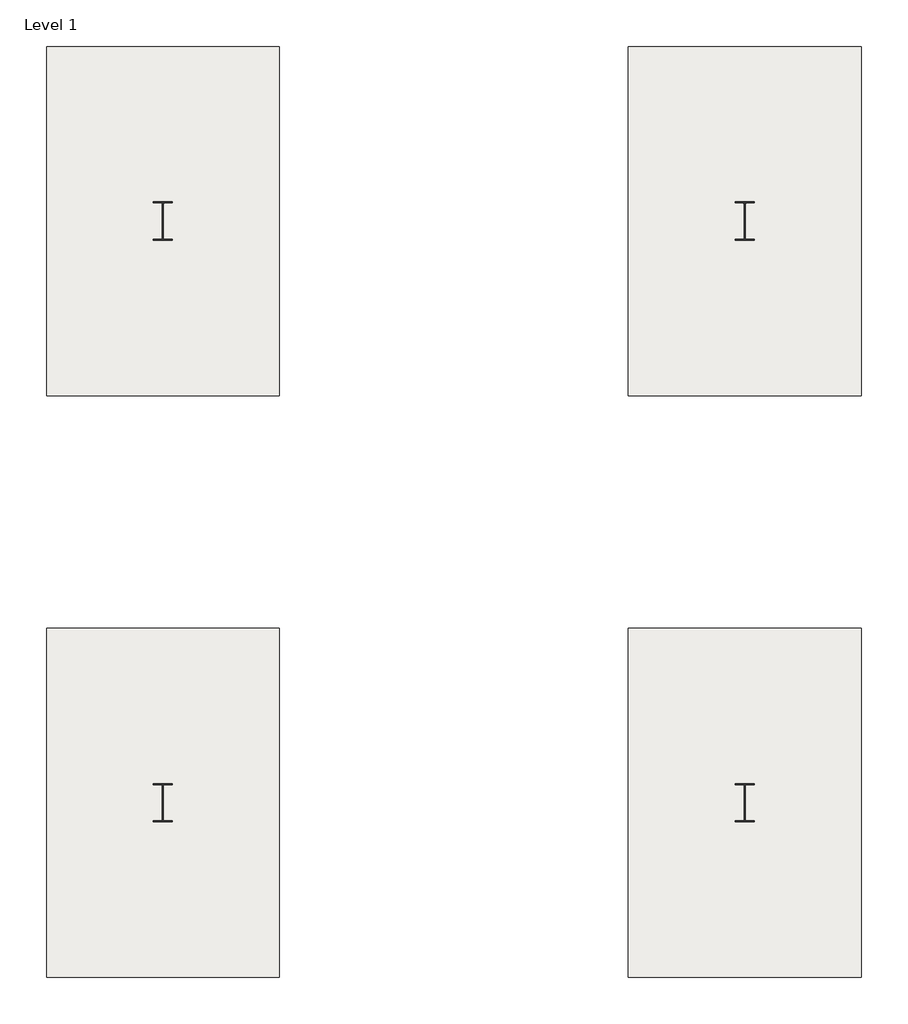
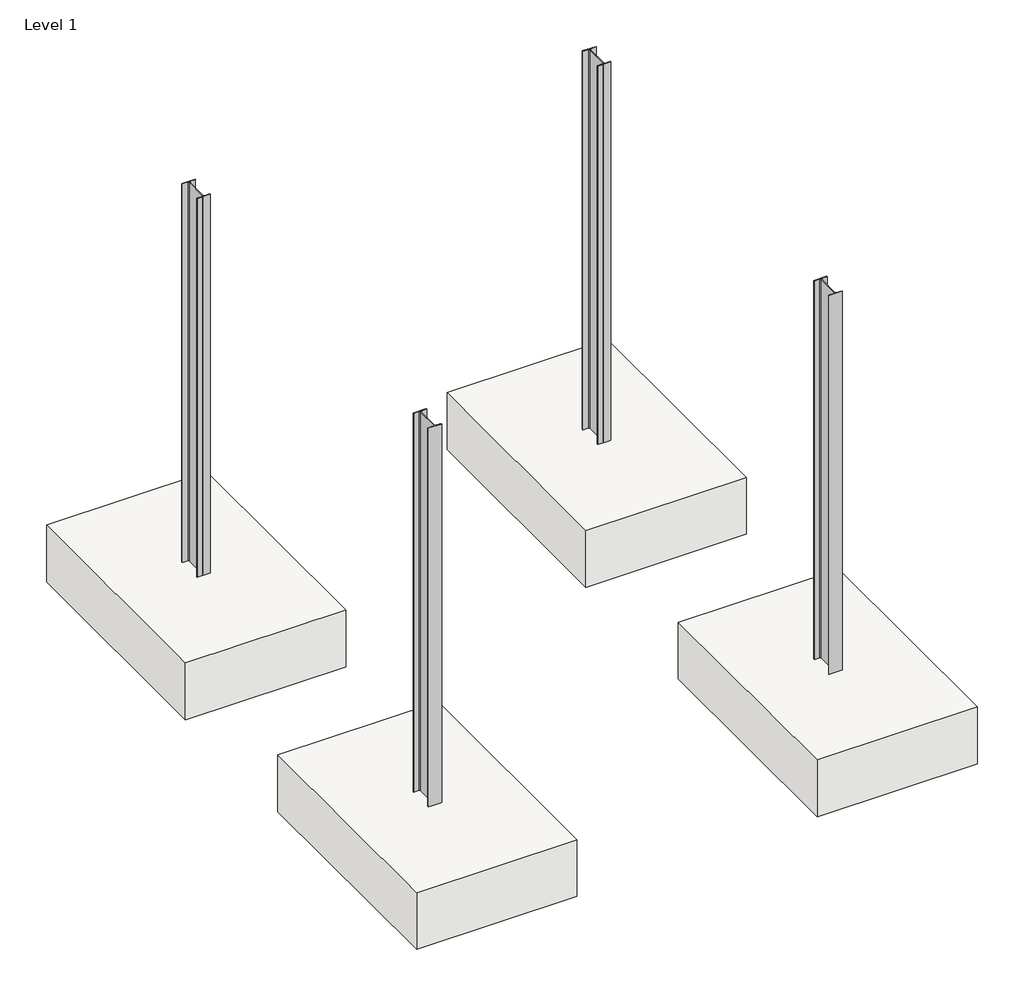
# One storey: 4 columns, 4 slabs.
"""IFC4 building model written with IfcOpenShell, lengths in millimetres."""

import ifcopenshell
import ifcopenshell.guid

model = None  # the IFC model being written
_history = None  # IfcOwnerHistory: only IFC2X3 demands one
_inside = {}  # id of a spatial element -> (the spatial element, [elements in it])
_under = {}  # id of a project, library or spatial element -> (it, [spatial elements below it])
_declared = {}  # id of a project -> (the project, [libraries it declares])
_typed = {}  # id of a type object -> (the type object, [elements of that type])
_made_of = {}  # id of a material, layer set ... -> (it, [elements and type objects made of it])


def new_model(schema):
    """Start an empty IFC model of exactly this schema.

    Asked for "IFC4X3", IfcOpenShell would pick the latest addendum, in which some entities
    have other attributes; the version numbers below select the first issue.
    IFC2X3 requires an IfcOwnerHistory on every rooted entity: one is made here for all.
    """
    global model, _history
    if schema == "IFC4X3":
        model = ifcopenshell.file(schema_version=(4, 3, 0, 0))
    else:
        model = ifcopenshell.file(schema=schema)
    _inside.clear()
    _under.clear()
    _declared.clear()
    _typed.clear()
    _made_of.clear()
    _history = None
    if model.schema == "IFC2X3":
        org = make("IfcOrganization", Name="unknown")
        user = make(
            "IfcPersonAndOrganization",
            ThePerson=make("IfcPerson", FamilyName="unknown"),
            TheOrganization=org,
        )
        app = make(
            "IfcApplication",
            ApplicationDeveloper=org,
            Version="unknown",
            ApplicationFullName="unknown",
            ApplicationIdentifier="unknown",
        )
        _history = make(
            "IfcOwnerHistory",
            OwningUser=user,
            OwningApplication=app,
            ChangeAction="ADDED",
            CreationDate=0,
        )
    return model


def make(cls, **values):
    """One entity of the class cls with the attributes given. An attribute that is None is left unset."""
    return model.create_entity(
        cls, **{name: value for name, value in values.items() if value is not None}
    )


def rooted(cls, **values):
    """An entity with a GlobalId (a new one), such as an element, a storey or a relation."""
    return make(cls, GlobalId=ifcopenshell.guid.new(), OwnerHistory=_history, **values)


def si_unit(unit_type, name, prefix=None):
    """IfcSIUnit, for example si_unit("LENGTHUNIT", "METRE", prefix="MILLI")."""
    return make("IfcSIUnit", UnitType=unit_type, Prefix=prefix, Name=name)


def assignment(units):
    """IfcUnitAssignment: the units of a project."""
    return None if units is None else make("IfcUnitAssignment", Units=units)


def point(xyz):
    """IfcCartesianPoint."""
    return None if xyz is None else make("IfcCartesianPoint", Coordinates=xyz)


def direction(xyz):
    """IfcDirection."""
    return None if xyz is None else make("IfcDirection", DirectionRatios=xyz)


def frame(location, z_axis=None, x_axis=None):
    """IfcAxis2Placement3D, a coordinate frame: its origin and axes. An axis left out is left unset."""
    return make(
        "IfcAxis2Placement3D",
        Location=point(location),
        Axis=direction(z_axis),
        RefDirection=direction(x_axis),
    )


def frame_2d(location, x_axis=None):
    """IfcAxis2Placement2D, a coordinate frame in the plane: its origin and x axis."""
    return make(
        "IfcAxis2Placement2D", Location=point(location), RefDirection=direction(x_axis)
    )


def origin():
    """The frame at (0, 0, 0) with its axes left unset."""
    return frame((0.0, 0.0, 0.0))


def origin_with_axes():
    """The frame at (0, 0, 0) with the z axis (0, 0, 1) and the x axis (1, 0, 0) written out."""
    return frame((0.0, 0.0, 0.0), z_axis=(0.0, 0.0, 1.0), x_axis=(1.0, 0.0, 0.0))


def place(relative_to, where):
    """IfcLocalPlacement: puts the frame where relative to a parent placement (None: the world)."""
    return make(
        "IfcLocalPlacement", PlacementRelTo=relative_to, RelativePlacement=where
    )


def context(
    kind, dimensions, precision=None, world=None, true_north=None, identifier=None
):
    """IfcGeometricRepresentationContext, for example the 3D "Model" context."""
    return make(
        "IfcGeometricRepresentationContext",
        ContextIdentifier=identifier,
        ContextType=kind,
        CoordinateSpaceDimension=dimensions,
        Precision=precision,
        WorldCoordinateSystem=world,
        TrueNorth=true_north,
    )


def project(units=None, contexts=None):
    """IfcProject with its units and contexts."""
    return rooted(
        "IfcProject",
        Name="project",
        RepresentationContexts=contexts,
        UnitsInContext=assignment(units),
    )


def spatial(cls, under=None, at=None, **own):
    """A site, building, storey or space (cls), placed at a placement, below another one or the project."""
    s = rooted(cls, ObjectPlacement=at, **own)
    if under is not None:
        _under.setdefault(under.id(), (under, []))[1].append(s)
    return s


def polyline(points):
    """IfcPolyline through the points."""
    return make("IfcPolyline", Points=[point(p) for p in points])


def circle_curve(where, radius):
    """IfcCircle in the frame where."""
    return make("IfcCircle", Position=where, Radius=radius)


def trimmed(basis, trim1, trim2, sense, master):
    """IfcTrimmedCurve: the piece of a basis curve between two trims."""
    return make(
        "IfcTrimmedCurve",
        BasisCurve=basis,
        Trim1=trim1,
        Trim2=trim2,
        SenseAgreement=sense,
        MasterRepresentation=master,
    )


def segment(curve, same_sense, transition):
    """IfcCompositeCurveSegment."""
    return make(
        "IfcCompositeCurveSegment",
        Transition=transition,
        SameSense=same_sense,
        ParentCurve=curve,
    )


def composite_curve(segments, self_intersect=None):
    """IfcCompositeCurve: segments joined end to end."""
    return make("IfcCompositeCurve", Segments=segments, SelfIntersect=self_intersect)


def outline(outer, holes=None, kind="AREA"):
    """IfcArbitraryClosedProfileDef: a profile drawn as a closed curve; with holes, ...WithVoids."""
    if holes is None:
        return make("IfcArbitraryClosedProfileDef", ProfileType=kind, OuterCurve=outer)
    return make(
        "IfcArbitraryProfileDefWithVoids",
        ProfileType=kind,
        OuterCurve=outer,
        InnerCurves=holes,
    )


def extrude(swept, where, along, depth):
    """IfcExtrudedAreaSolid: the profile swept, set in the frame where, extruded along a direction by depth."""
    return make(
        "IfcExtrudedAreaSolid",
        SweptArea=swept,
        Position=where,
        ExtrudedDirection=direction(along),
        Depth=depth,
    )


def shape(context_of_items, identifier, shape_type, items):
    """IfcShapeRepresentation: the items that make up one representation, for example the "Body"."""
    return make(
        "IfcShapeRepresentation",
        ContextOfItems=context_of_items,
        RepresentationIdentifier=identifier,
        RepresentationType=shape_type,
        Items=items,
    )


def source(mapping_origin, context_of_items, identifier, shape_type, items):
    """IfcRepresentationMap: a shape defined once, which mapped items show again and again."""
    return make(
        "IfcRepresentationMap",
        MappingOrigin=mapping_origin,
        MappedRepresentation=shape(context_of_items, identifier, shape_type, items),
    )


def transform(
    local_origin,
    x_axis=None,
    y_axis=None,
    z_axis=None,
    scale=None,
    scale2=None,
    scale3=None,
    uniform=True,
):
    """IfcCartesianTransformationOperator3D, or its non-uniform kind. x_axis, y_axis, z_axis: its Axis1, 2, 3."""
    if uniform:
        return make(
            "IfcCartesianTransformationOperator3D",
            Axis1=direction(x_axis),
            Axis2=direction(y_axis),
            LocalOrigin=point(local_origin),
            Scale=scale,
            Axis3=direction(z_axis),
        )
    return make(
        "IfcCartesianTransformationOperator3DnonUniform",
        Axis1=direction(x_axis),
        Axis2=direction(y_axis),
        LocalOrigin=point(local_origin),
        Scale=scale,
        Axis3=direction(z_axis),
        Scale2=scale2,
        Scale3=scale3,
    )


def mapped(mapping_source, mapping_target):
    """IfcMappedItem: shows the shape of a source again, moved by a transform."""
    return make(
        "IfcMappedItem", MappingSource=mapping_source, MappingTarget=mapping_target
    )


def made_of(thing, what):
    """Note that an element or type object is made of a material, layer set ...; save() writes the relation."""
    if what is not None:
        _made_of.setdefault(what.id(), (what, []))[1].append(thing)
    return thing


def element(
    cls,
    number,
    at=None,
    inside=None,
    cuts=None,
    type_object=None,
    material=None,
    context=None,
    identifier="Body",
    shape_type=None,
    held_by="IfcProductDefinitionShape",
    body=None,
    shapes=None,
    **own,
):
    """One element of the class cls, such as IfcWall. Its Tag is "e" and its number.

    at: its placement. inside: the storey or other place that contains it. cuts: it is an
    opening in that element (IfcRelVoidsElement). A single representation is given by context,
    identifier, shape_type and body (its items); several are given by shapes. held_by: the class
    of the entity that holds the representations. save() writes the other relations.
    """
    e = rooted(cls, Tag="e%d" % number, ObjectPlacement=at, **own)
    if body is not None:
        shapes = [shape(context, identifier, shape_type, body)]
    if shapes is not None:
        e.Representation = make(held_by, Representations=shapes)
    if inside is not None:
        _inside.setdefault(inside.id(), (inside, []))[1].append(e)
    if cuts is not None:
        rooted(
            "IfcRelVoidsElement", RelatingBuildingElement=cuts, RelatedOpeningElement=e
        )
    if type_object is not None:
        _typed.setdefault(type_object.id(), (type_object, []))[1].append(e)
    return made_of(e, material)


def aggregate(whole, parts):
    """IfcRelAggregates: a whole, such as a stair, and the parts it consists of."""
    return rooted("IfcRelAggregates", RelatingObject=whole, RelatedObjects=parts)


def save(model, path):
    """Write the relations noted so far, then the file.

    IfcRelAggregates (storeys below a building ...), IfcRelContainedInSpatialStructure (elements
    in a storey), IfcRelDefinesByType, IfcRelAssociatesMaterial and IfcRelDeclares: one each for
    every whole, place, type object, material and project.
    """
    for whole, parts in _under.values():
        aggregate(whole, parts)
    for where, things in _inside.values():
        rooted(
            "IfcRelContainedInSpatialStructure",
            RelatedElements=things,
            RelatingStructure=where,
        )
    for kind, things in _typed.values():
        rooted("IfcRelDefinesByType", RelatedObjects=things, RelatingType=kind)
    for what, things in _made_of.values():
        rooted("IfcRelAssociatesMaterial", RelatedObjects=things, RelatingMaterial=what)
    for by, libraries in _declared.values():
        rooted("IfcRelDeclares", RelatingContext=by, RelatedDefinitions=libraries)
    model.write(path)


def w_shapes_column_w8x10_fd6cb265(model_context):
    return source(origin(), model_context, "Body", "SweptSolid", [
        extrude(outline(composite_curve([segment(polyline([(50.038, 100.203), (50.038, 94.869), (9.779, 94.869)]), True, "CONTINUOUS"), segment(trimmed(circle_curve(frame_2d((9.779, 87.249)), 7.62), [point((9.779, 94.869))], [point((2.159, 87.249))], True, "CARTESIAN"), True, "CONTINUOUS"), segment(polyline([(2.159, 87.249), (2.159, -87.249)]), True, "CONTINUOUS"), segment(trimmed(circle_curve(frame_2d((9.779, -87.249)), 7.62), [point((2.159, -87.249))], [point((9.779, -94.869))], True, "CARTESIAN"), True, "CONTINUOUS"), segment(polyline([(9.779, -94.869), (50.038, -94.869), (50.038, -100.203), (-50.038, -100.203), (-50.038, -94.869), (-9.779, -94.869)]), True, "CONTINUOUS"), segment(trimmed(circle_curve(frame_2d((-9.779, -87.249)), 7.62), [point((-9.779, -94.869))], [point((-2.159, -87.249))], True, "CARTESIAN"), True, "CONTINUOUS"), segment(polyline([(-2.159, -87.249), (-2.159, 87.249)]), True, "CONTINUOUS"), segment(trimmed(circle_curve(frame_2d((-9.779, 87.249)), 7.62), [point((-2.159, 87.249))], [point((-9.779, 94.869))], True, "CARTESIAN"), True, "CONTINUOUS"), segment(polyline([(-9.779, 94.869), (-50.038, 94.869), (-50.038, 100.203), (50.038, 100.203)]), True, "CONTINUOUS")], self_intersect=False)), origin_with_axes(), (0.0, 0.0, 1.0), 3048.0),
    ])


def slab_5ba74754(model_context):
    return source(origin(), model_context, "Body", "SweptSolid", [
        extrude(outline(polyline([(609.6, 914.4), (609.6, -914.4), (-609.6, -914.4), (-609.6, 914.4), (609.6, 914.4)])), frame((0.0, 0.0, -457.2), z_axis=(0.0, 0.0, 1.0), x_axis=(1.0, 0.0, 0.0)), (0.0, 0.0, 1.0), 457.2),
    ])


model = new_model("IFC4")

# Units and contexts
model_context = context("Model", 3, world=origin())
ifc_project = project(units=[si_unit("LENGTHUNIT", "METRE", prefix="MILLI")], contexts=[model_context])

# Site, building, storey
site = spatial("IfcSite", under=ifc_project)
building = spatial("IfcBuilding", under=site)
storey = spatial("IfcBuildingStorey", under=building, Name="Level 1", Elevation=0.0)

# Columns
placement = place(None, origin())
w_shapes_column_w8x10_shape = w_shapes_column_w8x10_fd6cb265(model_context)
element("IfcColumn", 1, ObjectType="W Shapes-Column : W8X10", at=placement, inside=storey, context=model_context, shape_type="MappedRepresentation", body=[
    mapped(w_shapes_column_w8x10_shape, transform((3048.0, 0.0, 0.0), x_axis=(1.0, 0.0, 0.0), y_axis=(0.0, 1.0, 0.0), z_axis=(0.0, 0.0, 1.0))),
])
element("IfcColumn", 2, ObjectType="W Shapes-Column : W8X10", at=placement, inside=storey, context=model_context, shape_type="MappedRepresentation", body=[
    mapped(w_shapes_column_w8x10_shape, transform((3048.0, 3048.0, 0.0), x_axis=(1.0, 0.0, 0.0), y_axis=(0.0, 1.0, 0.0), z_axis=(0.0, 0.0, 1.0))),
])
element("IfcColumn", 3, ObjectType="W Shapes-Column : W8X10", at=placement, inside=storey, context=model_context, shape_type="MappedRepresentation", body=[
    mapped(w_shapes_column_w8x10_shape, transform((0.0, 3048.0, 0.0), x_axis=(1.0, 0.0, 0.0), y_axis=(0.0, 1.0, 0.0), z_axis=(0.0, 0.0, 1.0))),
])
element("IfcColumn", 4, ObjectType="W Shapes-Column : W8X10", at=placement, inside=storey, context=model_context, shape_type="MappedRepresentation", body=[
    mapped(w_shapes_column_w8x10_shape, transform((0.0, 0.0, 0.0), x_axis=(1.0, 0.0, 0.0), y_axis=(0.0, 1.0, 0.0), z_axis=(0.0, 0.0, 1.0))),
])

# Slabs
slab_shape = slab_5ba74754(model_context)
element("IfcSlab", 5, ObjectType="Footing-Rectangular : 72\" x 48\" x 18\"", at=placement, inside=storey, context=model_context, shape_type="MappedRepresentation", body=[
    mapped(slab_shape, transform((0.0, 3048.0, 0.0), x_axis=(1.0, 0.0, 0.0), y_axis=(0.0, 1.0, 0.0), z_axis=(0.0, 0.0, 1.0))),
])
element("IfcSlab", 6, ObjectType="Footing-Rectangular : 72\" x 48\" x 18\"", at=placement, inside=storey, context=model_context, shape_type="MappedRepresentation", body=[
    mapped(slab_shape, transform((3048.0, 3048.0, 0.0), x_axis=(1.0, 0.0, 0.0), y_axis=(0.0, 1.0, 0.0), z_axis=(0.0, 0.0, 1.0))),
])
element("IfcSlab", 7, ObjectType="Footing-Rectangular : 72\" x 48\" x 18\"", at=placement, inside=storey, context=model_context, shape_type="MappedRepresentation", body=[
    mapped(slab_shape, transform((3048.0, 0.0, 0.0), x_axis=(1.0, 0.0, 0.0), y_axis=(0.0, 1.0, 0.0), z_axis=(0.0, 0.0, 1.0))),
])
element("IfcSlab", 8, ObjectType="Footing-Rectangular : 72\" x 48\" x 18\"", at=placement, inside=storey, context=model_context, shape_type="MappedRepresentation", body=[
    mapped(slab_shape, transform((0.0, 0.0, 0.0), x_axis=(1.0, 0.0, 0.0), y_axis=(0.0, 1.0, 0.0), z_axis=(0.0, 0.0, 1.0))),
])

save(model, "model.ifc")

# Revit data of these elements
# Project information
#   Project Issue Date = "Issue Date"
#   Project Status = "Project Status"
#   Client Name = "Owner"
#   Project Address = "Enter address here"
#   Project Name = "Project Name"
#   Project Number = "Project Number"
# Grids (mm)
#   "1": line (0, 3382.905) -> (0, -500.676)
#   "2": line (3048, 3382.905) -> (3048, -500.676)
#   "B": line (3628.947, 0) -> (-577.435, 0)
#   "A": line (3628.947, 3048) -> (-577.435, 3048)
# Type "W Shapes-Column : W8X10"
#   Section Name Key = "W8x10"
#   Assembly Code = "B10"
#   Width = 100.076 mm
#   Web Thickness = 4.318 mm
#   Web Fillet = 7.62 mm
#   Warping Constant = 8297.76 cm⁶
#   Torsional Moment of Inertia = 1.77315 cm⁴
#   Section Area = 2.96 in²
#   Plastic Modulus weak axis = 0.000960648 (stored number, unit not read)
#   Plastic Modulus strong axis = 0.0051331 (stored number, unit not read)
#   Perimeter = 9.35736 m²/m
#   Nominal Weight = 145.939 N/m
#   Moment of Inertia weak axis = 86.9924 cm⁴
#   Moment of Inertia strong axis = 1281.99 cm⁴
#   Height = 200.406 mm
#   Flange Thickness = 5.334 mm
#   Elastic Modulus weak axis = 0.000613426 (stored number, unit not read)
#   Elastic Modulus strong axis = 0.00451968 (stored number, unit not read)
#   Centroid Vertical = 100.203 mm
#   Centroid Horizontal = 50.038 mm
#   Structural Material [instance default] = Steel ASTM A992
#   Principal Axes Angle = 0
# Type "Footing-Rectangular : 72\" x 48\" x 18\""
#   Assembly Code = "A1010100"
#   Width = 4' - 0"
#   Length = 6' - 0"
#   Thickness = 1' - 6"
#   Structural Material [instance default] = Concrete, Cast-in-Place gray
# Elements 1, 2, 3, 4 (IfcColumn, "W Shapes-Column : W8X10")
#   Comments = ""
#   Structural Material = Steel ASTM A992
#   Phase Created = New Construction
#   Materials on its faces: "Steel ASTM A992"
# Elements 5, 6, 7, 8 (IfcSlab, "Footing-Rectangular : 72\" x 48\" x 18\"")
#   Structural Material = Concrete, Cast-in-Place gray
#   Phase Created = New Construction
#   Materials on its faces: "Concrete, Cast-in-Place gray"
# Materials
#   "Steel ASTM A992": class "Metal", colour RGB 199 199 199, transparency 0, Description = "Structural steel 50ksi", Cost = 0
#   "Concrete, Cast-in-Place gray": class "Concrete", colour RGB 192 192 192, transparency 0, Description = "Cast-in-place concrete", Cost = 0
